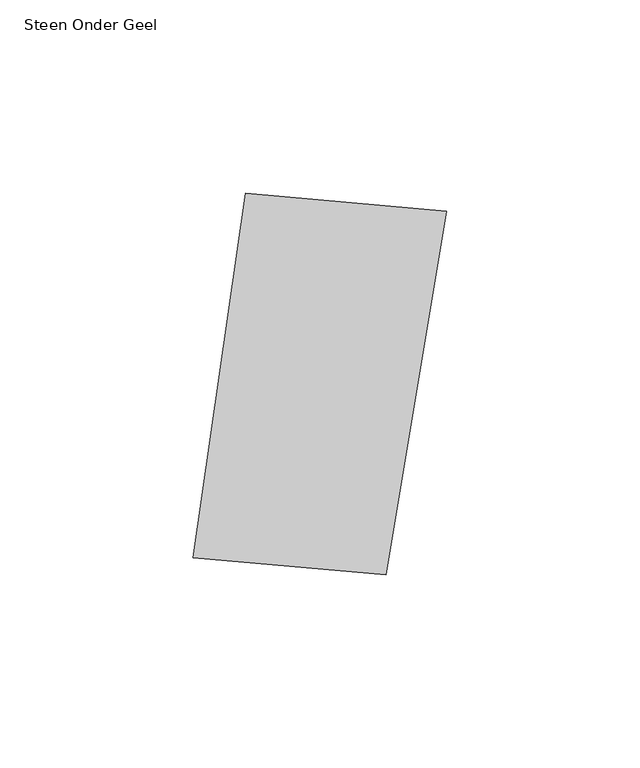
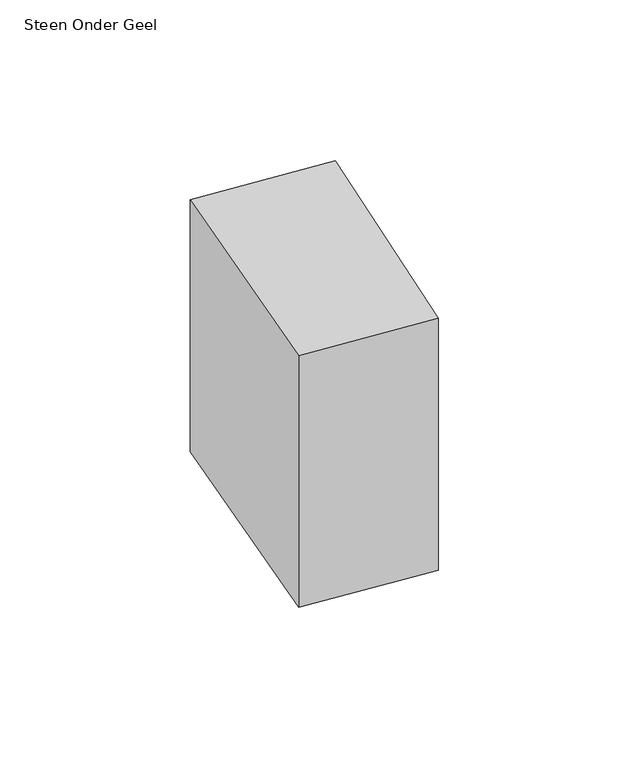
"""IFC4 building model written with IfcOpenShell, lengths in millimetres: proxy geometry, 00_GMA_steen_versie_4 : Steen Onder Geel."""

from ifc_helpers import new_model, si_unit, origin, origin_with_axes, place, context, project, spatial, polyline, outline, extrude, source, transform, mapped, element, save


def steen_onder_geel_67b0e7ce(model_context):
    return source(origin(), model_context, "Body", "SweptSolid", [
        extrude(outline(polyline([(108.0054294, 113.5688966), (92.3161243, 19.5677963), (42.5085422, 23.9501211), (56.093579, 118.1301694), (108.0054294, 113.5688966)])), origin_with_axes(), (0.0, 0.0, 1.0), 100.0),
    ])


if __name__ == "__main__":
    model = new_model("IFC4")
    model_context = context("Model", 3, world=origin())
    ifc_project = project(units=[si_unit("LENGTHUNIT", "METRE", prefix="MILLI")], contexts=[model_context])
    site = spatial("IfcSite", under=ifc_project)
    building = spatial("IfcBuilding", under=site)
    placement = place(None, origin())
    steen_onder_geel_shape = steen_onder_geel_67b0e7ce(model_context)
    element("IfcBuildingElementProxy", 1, Name="00_GMA_steen_versie_4 : Steen Onder Geel", ObjectType="00_GMA_steen_versie_4 : Steen Onder Geel", at=placement, inside=building, context=model_context, shape_type="MappedRepresentation", body=[
        mapped(steen_onder_geel_shape, transform((0.0, 0.0, 0.0), x_axis=(1.0, 0.0, 0.0), y_axis=(0.0, 1.0, 0.0), z_axis=(0.0, 0.0, 1.0))),
    ])
    save(model, "model.ifc")

# Revit data of these elements
# Type "00_GMA_steen_versie_4 : Steen Onder Geel"
#   StootVoegHalfBoven [instance default] = 5 mm
#   StootVoegHalf [instance default] = 5 mm
#   StootVoegBreedteOnder = 10 mm
#   StootVoegBreedteBoven = 10 mm
#   Steendikte = 100 mm
#   LintVoegOnderHalf = 0 mm
#   LintVoegOnder = 0 mm
#   LintVoegBovenHalf = 5 mm
#   LintVoegBoven = 10 mm
#   materiaal = 21_steen_geel
#   MateriaalVoeg = none
#   Default Elevation = 0
# Element 1 (IfcBuildingElementProxy, "00_GMA_steen_versie_4 : Steen Onder Geel")
#   Materials on its faces: "21_steen_geel"
# Materials
#   "21_steen_geel": class "Unassigned", colour RGB 202 202 0, transparency 0, Cost = 0
